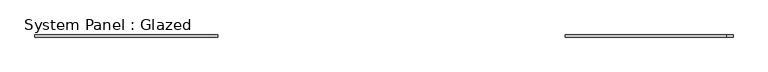
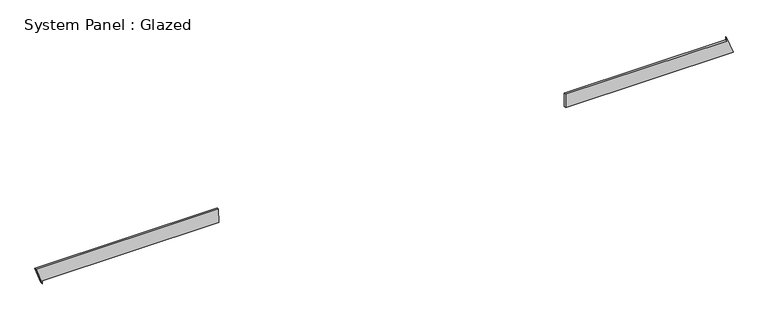
"""IFC4 building model written with IfcOpenShell, lengths in millimetres: plate geometry, System Panel : Glazed."""

from ifc_helpers import new_model, si_unit, frame, origin, place, context, project, spatial, polyline, outline, extrude, source, transform, mapped, element, save


def system_panel_glazed_79f041e2(model_context):
    return source(origin(), model_context, "Body", "SweptSolid", [
        extrude(outline(polyline([(0.0, -3956.878339), (35.3553391, -3956.878339), (35.3553391, -1917.9130986), (198.6893709, -1919.9548357), (198.7125272, -4027.1816216), (0.0, -3956.878339)])), frame((0.0, -49.5, 0.0), z_axis=(0.0, 1.0, 0.0), x_axis=(0.0, 0.0, 1.0)), (0.0, 0.0, 1.0), 25.0),
        extrude(outline(polyline([(35.3553391, 2090.7206202), (35.3553391, 4027.1816216), (233.9801319, 3956.6725023), (198.6247928, 3956.6721138), (198.6452733, 2092.942533), (35.3553391, 2090.7206202)])), frame((0.0, -49.5, 0.0), z_axis=(0.0, 1.0, 0.0), x_axis=(0.0, 0.0, 1.0)), (0.0, 0.0, 1.0), 25.0),
    ])


if __name__ == "__main__":
    model = new_model("IFC4")
    model_context = context("Model", 3, world=origin())
    ifc_project = project(units=[si_unit("LENGTHUNIT", "METRE", prefix="MILLI")], contexts=[model_context])
    site = spatial("IfcSite", under=ifc_project)
    building = spatial("IfcBuilding", under=site)
    placement = place(None, origin())
    system_panel_glazed_shape = system_panel_glazed_79f041e2(model_context)
    element("IfcPlate", 1, ObjectType="System Panel : Glazed", at=placement, inside=building, context=model_context, shape_type="MappedRepresentation", body=[
        mapped(system_panel_glazed_shape, transform((0.0, 0.0, 0.0), x_axis=(1.0, 0.0, 0.0), y_axis=(0.0, 1.0, 0.0), z_axis=(0.0, 0.0, 1.0))),
    ])
    save(model, "model.ifc")

# Revit data of these elements
# Element 1 (IfcPlate, "System Panel : Glazed")
#   Materials on its faces: "Glass"
# Materials
#   "Glass": class "Glass", colour RGB 218 227 224, transparency 0.85, Description = "Soda Lime Glass", Cost = 0
